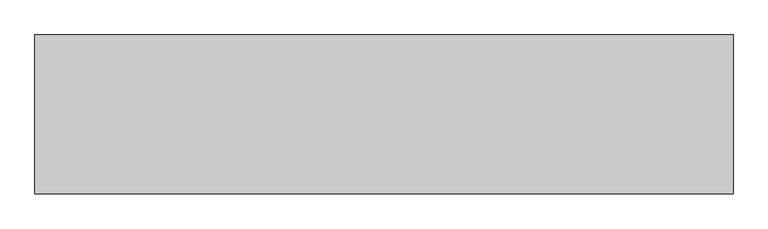
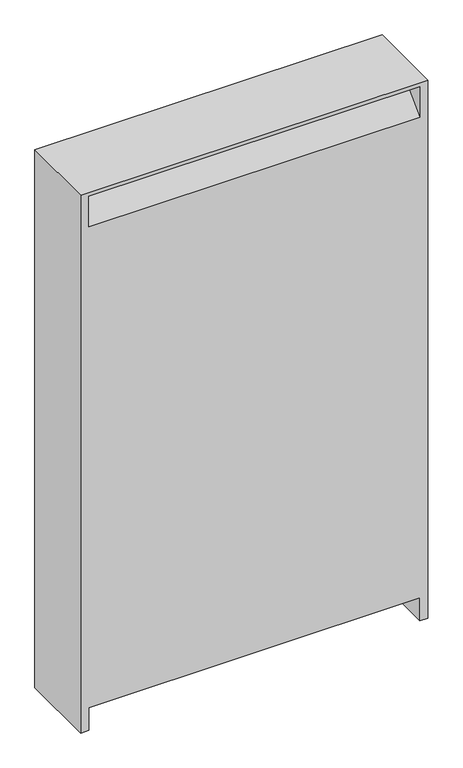
"""IFC4 building model written with IfcOpenShell, lengths in millimetres: proxy geometry, Dry Type Transformer - 480-208Y120 - NEMA Type 2 : Small Power Sub-Dist Board."""

from ifc_helpers import new_model, si_unit, origin, place, context, project, spatial, faceted_brep, source, transform, mapped, element, save


def electrical_equipment_6f0a50c8(model_context):
    return source(origin(), model_context, "Body", "Brep", [
        faceted_brep([(550.0, 134.7158651, 1800.0), (550.0, 384.7158651, 1800.0), (-550.0, 384.7158651, 1800.0), (-550.0, 134.7158651, 1800.0), (-550.0, 134.7158651, 0.0), (-550.0, 384.7158651, 0.0), (-524.6, 384.7158651, 0.0), (-524.6, 134.7158651, 0.0), (550.0, 384.7158651, 0.0), (550.0, 134.7158651, 0.0), (524.6, 134.7158651, 0.0), (524.6, 384.7158651, 0.0), (524.6, 384.7158651, 76.2), (-524.6, 384.7158651, 76.2), (524.6, 384.7158651, 1685.7), (524.6, 384.7158651, 1787.3), (-524.6, 384.7158651, 1787.3), (-524.6, 384.7158651, 1685.7), (-524.6, 134.7158651, 76.2), (524.6, 134.7158651, 76.2), (524.6, 134.7158651, 1787.3), (524.6, 134.7158651, 1685.7), (-524.6, 134.7158651, 1685.7), (-524.6, 134.7158651, 1787.3), (524.6, 236.3158651, 1787.3), (-524.6, 236.3158651, 1787.3), (524.6, 283.1158651, 1787.3), (-524.6, 283.1158651, 1787.3)], [[[0, 1, 2, 3]], [[4, 5, 6, 7]], [[8, 9, 10, 11]], [[1, 0, 9, 8]], [[2, 1, 8, 11, 12, 13, 6, 5], [14, 15, 16, 17]], [[3, 2, 5, 4]], [[0, 3, 4, 7, 18, 19, 10, 9], [20, 21, 22, 23]], [[18, 13, 12, 19]], [[13, 18, 7, 6]], [[19, 12, 11, 10]], [[24, 21, 20]], [[25, 23, 22]], [[24, 20, 23, 25]], [[21, 24, 25, 22]], [[26, 15, 14]], [[27, 17, 16]], [[26, 14, 17, 27]], [[15, 26, 27, 16]]]),
    ])


if __name__ == "__main__":
    model = new_model("IFC4")
    model_context = context("Model", 3, world=origin())
    ifc_project = project(units=[si_unit("LENGTHUNIT", "METRE", prefix="MILLI")], contexts=[model_context])
    site = spatial("IfcSite", under=ifc_project)
    building = spatial("IfcBuilding", under=site)
    placement = place(None, origin())
    electrical_equipment_shape = electrical_equipment_6f0a50c8(model_context)
    element("IfcBuildingElementProxy", 1, Name="Dry Type Transformer - 480-208Y120 - NEMA Type 2 : Small Power Sub-Dist Board", ObjectType="Dry Type Transformer - 480-208Y120 - NEMA Type 2 : Small Power Sub-Dist Board", at=placement, inside=building, context=model_context, shape_type="MappedRepresentation", body=[
        mapped(electrical_equipment_shape, transform((0.0, 0.0, 0.0), x_axis=(1.0, 0.0, 0.0), y_axis=(0.0, 1.0, 0.0), z_axis=(0.0, 0.0, 1.0))),
    ])
    save(model, "model.ifc")

# Revit data of these elements
# Type "Dry Type Transformer - 480-208Y120 - NEMA Type 2 : Small Power Sub-Dist Board"
#   built-in parameter 1140083 [instance default] = "Type 2"
#   Transformer Length = 1100 mm
#   Primary Voltage = 480 V
#   Transformer Height = 1800 mm
#   built-in parameter 1140140 [instance default] = 1 (stored number, unit not read)
#   Transformer Width = 250 mm
#   built-in parameter 1140142 [instance default] = -1
#   Primary Number of Poles = 3
#   built-in parameter 1140079 [instance default] = 3
#   Transformer Material = none
#   Load Classification = Transformer
#   Default Elevation = 0
#   Assembly Code = ""
#   built-in parameter 1140087 [instance default] = 1
